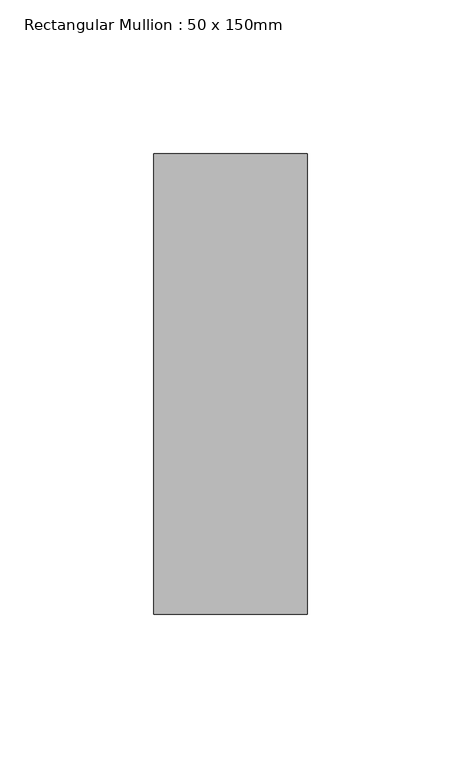
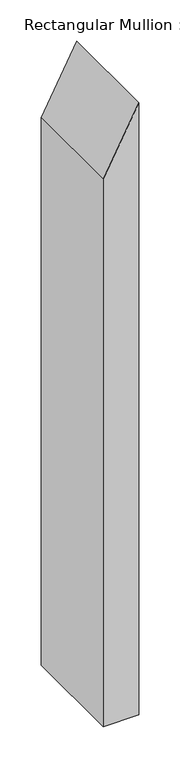
"""IFC4 building model written with IfcOpenShell, lengths in millimetres: member geometry, Rectangular Mullion : 50 x 150mm."""

from ifc_helpers import new_model, si_unit, frame, origin, place, context, project, spatial, polyline, outline, extrude, source, transform, mapped, element, save


def rectangular_mullion_50_x_150mm_bc447247(model_context):
    return source(origin(), model_context, "Body", "SweptSolid", [
        extrude(outline(polyline([(0.0, 0.0), (-96.0491063, -50.0), (-907.1712646, -50.0), (-907.1712646, 0.0), (0.0, 0.0)])), frame((0.0, -75.0, 0.0), z_axis=(0.0, 1.0, 0.0), x_axis=(0.0, 0.0, 1.0)), (0.0, 0.0, 1.0), 150.0),
    ])


if __name__ == "__main__":
    model = new_model("IFC4")
    model_context = context("Model", 3, world=origin())
    ifc_project = project(units=[si_unit("LENGTHUNIT", "METRE", prefix="MILLI")], contexts=[model_context])
    site = spatial("IfcSite", under=ifc_project)
    building = spatial("IfcBuilding", under=site)
    placement = place(None, origin())
    rectangular_mullion_50_x_150mm_shape = rectangular_mullion_50_x_150mm_bc447247(model_context)
    element("IfcMember", 1, ObjectType="Rectangular Mullion : 50 x 150mm", at=placement, inside=building, context=model_context, shape_type="MappedRepresentation", body=[
        mapped(rectangular_mullion_50_x_150mm_shape, transform((0.0, 0.0, 0.0), x_axis=(1.0, 0.0, 0.0), y_axis=(0.0, 1.0, 0.0), z_axis=(0.0, 0.0, 1.0))),
    ])
    save(model, "model.ifc")

# Revit data of these elements
# Type "Rectangular Mullion : 50 x 150mm"
#   built-in parameter 1007304 = 0.492126 (stored number, unit not read)
#   built-in parameter 1007301 = 0.082021 (stored number, unit not read)
#   built-in parameter 1007300 = 0.082021 (stored number, unit not read)
# Element 1 (IfcMember, "Rectangular Mullion : 50 x 150mm")
#   Materials on its faces: "Aluminium"
# Materials
#   "Aluminium": class "Metal", colour RGB 247 247 247, transparency 0, Description = "Aluminium 6061", Cost = 0
